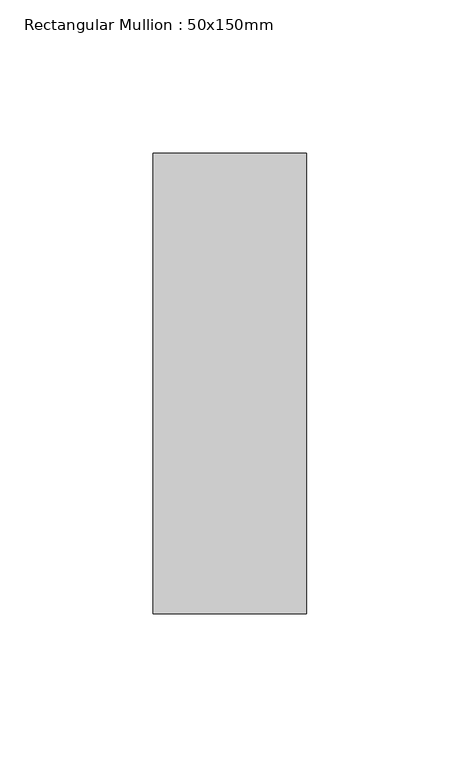
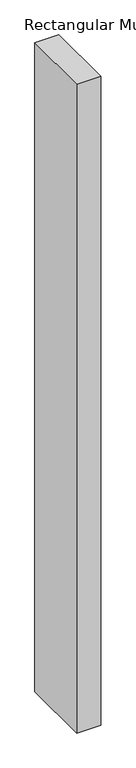
"""IFC4 building model written with IfcOpenShell, lengths in millimetres: member geometry, Rectangular Mullion : 50x150mm."""

import ifcopenshell
import ifcopenshell.guid

model = None  # the IFC model being written
_history = None  # IfcOwnerHistory: only IFC2X3 demands one
_inside = {}  # id of a spatial element -> (the spatial element, [elements in it])
_under = {}  # id of a project, library or spatial element -> (it, [spatial elements below it])
_declared = {}  # id of a project -> (the project, [libraries it declares])
_typed = {}  # id of a type object -> (the type object, [elements of that type])
_made_of = {}  # id of a material, layer set ... -> (it, [elements and type objects made of it])


def new_model(schema):
    """Start an empty IFC model of exactly this schema.

    Asked for "IFC4X3", IfcOpenShell would pick the latest addendum, in which some entities
    have other attributes; the version numbers below select the first issue.
    IFC2X3 requires an IfcOwnerHistory on every rooted entity: one is made here for all.
    """
    global model, _history
    if schema == "IFC4X3":
        model = ifcopenshell.file(schema_version=(4, 3, 0, 0))
    else:
        model = ifcopenshell.file(schema=schema)
    _inside.clear()
    _under.clear()
    _declared.clear()
    _typed.clear()
    _made_of.clear()
    _history = None
    if model.schema == "IFC2X3":
        org = make("IfcOrganization", Name="unknown")
        user = make(
            "IfcPersonAndOrganization",
            ThePerson=make("IfcPerson", FamilyName="unknown"),
            TheOrganization=org,
        )
        app = make(
            "IfcApplication",
            ApplicationDeveloper=org,
            Version="unknown",
            ApplicationFullName="unknown",
            ApplicationIdentifier="unknown",
        )
        _history = make(
            "IfcOwnerHistory",
            OwningUser=user,
            OwningApplication=app,
            ChangeAction="ADDED",
            CreationDate=0,
        )
    return model


def make(cls, **values):
    """One entity of the class cls with the attributes given. An attribute that is None is left unset."""
    return model.create_entity(
        cls, **{name: value for name, value in values.items() if value is not None}
    )


def rooted(cls, **values):
    """An entity with a GlobalId (a new one), such as an element, a storey or a relation."""
    return make(cls, GlobalId=ifcopenshell.guid.new(), OwnerHistory=_history, **values)


def si_unit(unit_type, name, prefix=None):
    """IfcSIUnit, for example si_unit("LENGTHUNIT", "METRE", prefix="MILLI")."""
    return make("IfcSIUnit", UnitType=unit_type, Prefix=prefix, Name=name)


def assignment(units):
    """IfcUnitAssignment: the units of a project."""
    return None if units is None else make("IfcUnitAssignment", Units=units)


def point(xyz):
    """IfcCartesianPoint."""
    return None if xyz is None else make("IfcCartesianPoint", Coordinates=xyz)


def direction(xyz):
    """IfcDirection."""
    return None if xyz is None else make("IfcDirection", DirectionRatios=xyz)


def frame(location, z_axis=None, x_axis=None):
    """IfcAxis2Placement3D, a coordinate frame: its origin and axes. An axis left out is left unset."""
    return make(
        "IfcAxis2Placement3D",
        Location=point(location),
        Axis=direction(z_axis),
        RefDirection=direction(x_axis),
    )


def origin():
    """The frame at (0, 0, 0) with its axes left unset."""
    return frame((0.0, 0.0, 0.0))


def place(relative_to, where):
    """IfcLocalPlacement: puts the frame where relative to a parent placement (None: the world)."""
    return make(
        "IfcLocalPlacement", PlacementRelTo=relative_to, RelativePlacement=where
    )


def context(
    kind, dimensions, precision=None, world=None, true_north=None, identifier=None
):
    """IfcGeometricRepresentationContext, for example the 3D "Model" context."""
    return make(
        "IfcGeometricRepresentationContext",
        ContextIdentifier=identifier,
        ContextType=kind,
        CoordinateSpaceDimension=dimensions,
        Precision=precision,
        WorldCoordinateSystem=world,
        TrueNorth=true_north,
    )


def project(units=None, contexts=None):
    """IfcProject with its units and contexts."""
    return rooted(
        "IfcProject",
        Name="project",
        RepresentationContexts=contexts,
        UnitsInContext=assignment(units),
    )


def spatial(cls, under=None, at=None, **own):
    """A site, building, storey or space (cls), placed at a placement, below another one or the project."""
    s = rooted(cls, ObjectPlacement=at, **own)
    if under is not None:
        _under.setdefault(under.id(), (under, []))[1].append(s)
    return s


def polyline(points):
    """IfcPolyline through the points."""
    return make("IfcPolyline", Points=[point(p) for p in points])


def outline(outer, holes=None, kind="AREA"):
    """IfcArbitraryClosedProfileDef: a profile drawn as a closed curve; with holes, ...WithVoids."""
    if holes is None:
        return make("IfcArbitraryClosedProfileDef", ProfileType=kind, OuterCurve=outer)
    return make(
        "IfcArbitraryProfileDefWithVoids",
        ProfileType=kind,
        OuterCurve=outer,
        InnerCurves=holes,
    )


def extrude(swept, where, along, depth):
    """IfcExtrudedAreaSolid: the profile swept, set in the frame where, extruded along a direction by depth."""
    return make(
        "IfcExtrudedAreaSolid",
        SweptArea=swept,
        Position=where,
        ExtrudedDirection=direction(along),
        Depth=depth,
    )


def shape(context_of_items, identifier, shape_type, items):
    """IfcShapeRepresentation: the items that make up one representation, for example the "Body"."""
    return make(
        "IfcShapeRepresentation",
        ContextOfItems=context_of_items,
        RepresentationIdentifier=identifier,
        RepresentationType=shape_type,
        Items=items,
    )


def source(mapping_origin, context_of_items, identifier, shape_type, items):
    """IfcRepresentationMap: a shape defined once, which mapped items show again and again."""
    return make(
        "IfcRepresentationMap",
        MappingOrigin=mapping_origin,
        MappedRepresentation=shape(context_of_items, identifier, shape_type, items),
    )


def transform(
    local_origin,
    x_axis=None,
    y_axis=None,
    z_axis=None,
    scale=None,
    scale2=None,
    scale3=None,
    uniform=True,
):
    """IfcCartesianTransformationOperator3D, or its non-uniform kind. x_axis, y_axis, z_axis: its Axis1, 2, 3."""
    if uniform:
        return make(
            "IfcCartesianTransformationOperator3D",
            Axis1=direction(x_axis),
            Axis2=direction(y_axis),
            LocalOrigin=point(local_origin),
            Scale=scale,
            Axis3=direction(z_axis),
        )
    return make(
        "IfcCartesianTransformationOperator3DnonUniform",
        Axis1=direction(x_axis),
        Axis2=direction(y_axis),
        LocalOrigin=point(local_origin),
        Scale=scale,
        Axis3=direction(z_axis),
        Scale2=scale2,
        Scale3=scale3,
    )


def mapped(mapping_source, mapping_target):
    """IfcMappedItem: shows the shape of a source again, moved by a transform."""
    return make(
        "IfcMappedItem", MappingSource=mapping_source, MappingTarget=mapping_target
    )


def made_of(thing, what):
    """Note that an element or type object is made of a material, layer set ...; save() writes the relation."""
    if what is not None:
        _made_of.setdefault(what.id(), (what, []))[1].append(thing)
    return thing


def element(
    cls,
    number,
    at=None,
    inside=None,
    cuts=None,
    type_object=None,
    material=None,
    context=None,
    identifier="Body",
    shape_type=None,
    held_by="IfcProductDefinitionShape",
    body=None,
    shapes=None,
    **own,
):
    """One element of the class cls, such as IfcWall. Its Tag is "e" and its number.

    at: its placement. inside: the storey or other place that contains it. cuts: it is an
    opening in that element (IfcRelVoidsElement). A single representation is given by context,
    identifier, shape_type and body (its items); several are given by shapes. held_by: the class
    of the entity that holds the representations. save() writes the other relations.
    """
    e = rooted(cls, Tag="e%d" % number, ObjectPlacement=at, **own)
    if body is not None:
        shapes = [shape(context, identifier, shape_type, body)]
    if shapes is not None:
        e.Representation = make(held_by, Representations=shapes)
    if inside is not None:
        _inside.setdefault(inside.id(), (inside, []))[1].append(e)
    if cuts is not None:
        rooted(
            "IfcRelVoidsElement", RelatingBuildingElement=cuts, RelatedOpeningElement=e
        )
    if type_object is not None:
        _typed.setdefault(type_object.id(), (type_object, []))[1].append(e)
    return made_of(e, material)


def aggregate(whole, parts):
    """IfcRelAggregates: a whole, such as a stair, and the parts it consists of."""
    return rooted("IfcRelAggregates", RelatingObject=whole, RelatedObjects=parts)


def save(model, path):
    """Write the relations noted so far, then the file.

    IfcRelAggregates (storeys below a building ...), IfcRelContainedInSpatialStructure (elements
    in a storey), IfcRelDefinesByType, IfcRelAssociatesMaterial and IfcRelDeclares: one each for
    every whole, place, type object, material and project.
    """
    for whole, parts in _under.values():
        aggregate(whole, parts)
    for where, things in _inside.values():
        rooted(
            "IfcRelContainedInSpatialStructure",
            RelatedElements=things,
            RelatingStructure=where,
        )
    for kind, things in _typed.values():
        rooted("IfcRelDefinesByType", RelatedObjects=things, RelatingType=kind)
    for what, things in _made_of.values():
        rooted("IfcRelAssociatesMaterial", RelatedObjects=things, RelatingMaterial=what)
    for by, libraries in _declared.values():
        rooted("IfcRelDeclares", RelatingContext=by, RelatedDefinitions=libraries)
    model.write(path)


def rectangular_mullion_50x150mm_acb4c03f(model_context):
    return source(origin(), model_context, "Body", "SweptSolid", [
        extrude(outline(polyline([(25.0, 75.0), (25.0, -75.0), (-25.0, -75.0), (-25.0, 75.0), (25.0, 75.0)])), frame((0.0, 0.0, -1425.0000002), z_axis=(0.0, 0.0, 1.0), x_axis=(1.0, 0.0, 0.0)), (0.0, 0.0, 1.0), 1425.0000002),
    ])


if __name__ == "__main__":
    model = new_model("IFC4")
    model_context = context("Model", 3, world=origin())
    ifc_project = project(units=[si_unit("LENGTHUNIT", "METRE", prefix="MILLI")], contexts=[model_context])
    site = spatial("IfcSite", under=ifc_project)
    building = spatial("IfcBuilding", under=site)
    placement = place(None, origin())
    rectangular_mullion_50x150mm_shape = rectangular_mullion_50x150mm_acb4c03f(model_context)
    element("IfcMember", 1, ObjectType="Rectangular Mullion : 50x150mm", at=placement, inside=building, context=model_context, shape_type="MappedRepresentation", body=[
        mapped(rectangular_mullion_50x150mm_shape, transform((0.0, 0.0, 0.0), x_axis=(1.0, 0.0, 0.0), y_axis=(0.0, 1.0, 0.0), z_axis=(0.0, 0.0, 1.0))),
    ])
    save(model, "model.ifc")

# Revit data of these elements
# Type "Rectangular Mullion : 50x150mm"
#   Keynote = "H11"
#   built-in parameter 1007304 = 0.492126 (stored number, unit not read)
#   built-in parameter 1007301 = 0.082021 (stored number, unit not read)
#   built-in parameter 1007300 = 0.082021 (stored number, unit not read)
# Element 1 (IfcMember, "Rectangular Mullion : 50x150mm")
#   Materials on its faces: "Aluminium"
# Materials
#   "Aluminium": class "Metal", colour RGB 247 247 247, transparency 0, Description = "Aluminium 6061", Cost = 0
